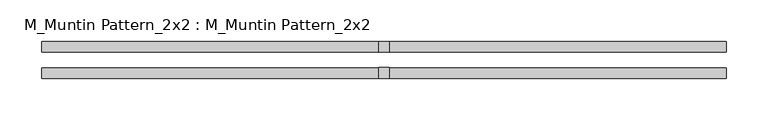
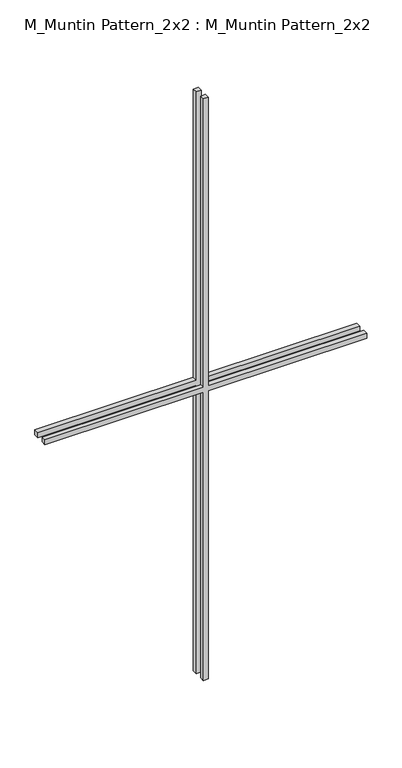
"""IFC4 building model written with IfcOpenShell, lengths in millimetres: proxy geometry, M_Muntin Pattern_2x2 : M_Muntin Pattern_2x2."""

from ifc_helpers import new_model, si_unit, frame, origin, place, context, project, spatial, polyline, outline, extrude, source, transform, mapped, element, save


def m_muntin_pattern_2x2_m_muntin_pattern_2x2_65db4d50(model_context):
    return source(origin(), model_context, "Body", "SweptSolid", [
        extrude(outline(polyline([(793.25, -6.35), (793.25, -411.9), (780.55, -411.9), (780.55, -6.35), (0.0, -6.35), (0.0, 6.35), (780.55, 6.35), (780.55, 411.9), (793.25, 411.9), (793.25, 6.35), (1573.8, 6.35), (1573.8, -6.35), (793.25, -6.35)])), frame((0.0, -22.225, 0.0), z_axis=(0.0, 1.0, 0.0), x_axis=(0.0, 0.0, 1.0)), (0.0, 0.0, 1.0), 12.7),
        extrude(outline(polyline([(793.25, -6.35), (793.25, -411.9), (780.55, -411.9), (780.55, -6.35), (0.0, -6.35), (0.0, 6.35), (780.55, 6.35), (780.55, 411.9), (793.25, 411.9), (793.25, 6.35), (1573.8, 6.35), (1573.8, -6.35), (793.25, -6.35)])), frame((0.0, 9.525, 0.0), z_axis=(0.0, 1.0, 0.0), x_axis=(0.0, 0.0, 1.0)), (0.0, 0.0, 1.0), 12.7),
    ])


if __name__ == "__main__":
    model = new_model("IFC4")
    model_context = context("Model", 3, world=origin())
    ifc_project = project(units=[si_unit("LENGTHUNIT", "METRE", prefix="MILLI")], contexts=[model_context])
    site = spatial("IfcSite", under=ifc_project)
    building = spatial("IfcBuilding", under=site)
    placement = place(None, origin())
    m_muntin_pattern_2x2_m_muntin_pattern_2x2_shape = m_muntin_pattern_2x2_m_muntin_pattern_2x2_65db4d50(model_context)
    element("IfcBuildingElementProxy", 1, Name="M_Muntin Pattern_2x2 : M_Muntin Pattern_2x2", ObjectType="M_Muntin Pattern_2x2 : M_Muntin Pattern_2x2", at=placement, inside=building, context=model_context, shape_type="MappedRepresentation", body=[
        mapped(m_muntin_pattern_2x2_m_muntin_pattern_2x2_shape, transform((0.0, 0.0, 0.0), x_axis=(1.0, 0.0, 0.0), y_axis=(0.0, 1.0, 0.0), z_axis=(0.0, 0.0, 1.0))),
    ])
    save(model, "model.ifc")

# Revit data of these elements
# Type "M_Muntin Pattern_2x2 : M_Muntin Pattern_2x2"
#   Width [instance default] = 1200 mm
#   Thickness = 12.7 mm
#   Height [instance default] = 1200 mm
#   Distance = 19.05 mm
#   Interior Material [instance default] = none
#   Exterior Material [instance default] = none
#   Default Elevation = 0
# Element 1 (IfcBuildingElementProxy, "M_Muntin Pattern_2x2 : M_Muntin Pattern_2x2")
#   Width = 823.8 mm
#   Height = 1573.8 mm
#   Interior Material = Wood - Stained
#   Exterior Material = Clad - White
#   Materials on its faces: "Clad - White", "Wood - Stained"
# Materials
#   "Clad - White": class "Wood", colour RGB 245 245 243, transparency 0, Cost = 0
#   "Wood - Stained": class "Wood", colour RGB 173 132 96, transparency 0, Cost = 0
